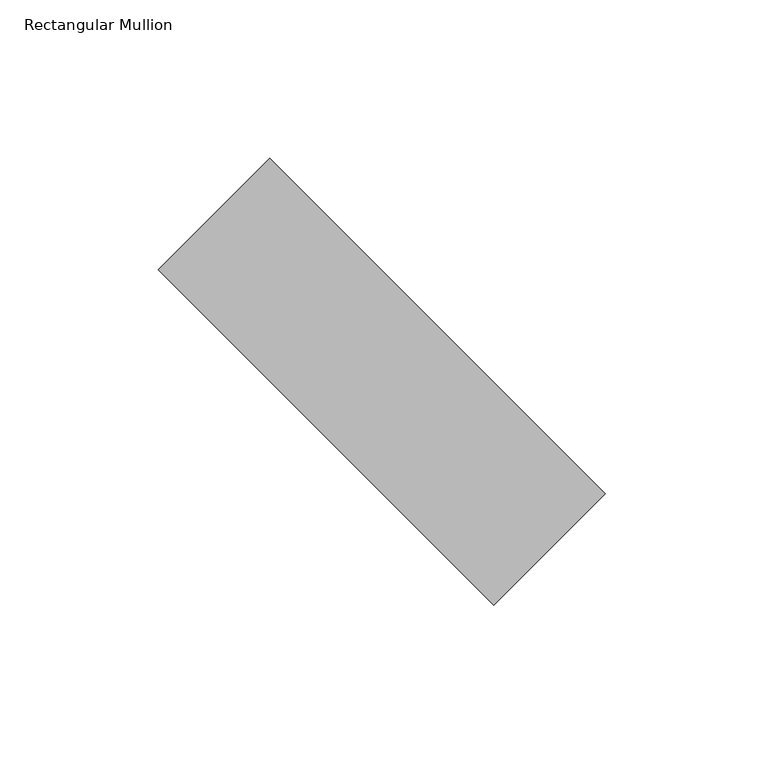
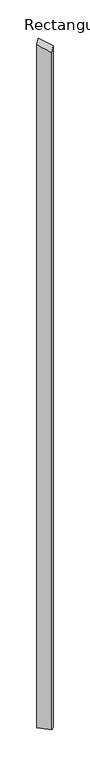
"""IFC4 building model written with IfcOpenShell, lengths in millimetres: member geometry, Rectangular Mullion : tilted mullions."""

from ifc_helpers import new_model, si_unit, origin, place, context, project, spatial, faceted_brep, source, transform, mapped, element, save


def rectangular_mullion_5ef0547a(model_context):
    return source(origin(), model_context, "Body", "Brep", [
        faceted_brep([(-35.3553391, 70.7106781, -7999.4591801), (70.7106781, -35.3553391, -7999.4591801), (35.3553391, -70.7106781, -7999.4591801), (-70.7106781, 35.3553391, -7999.4591801), (-70.7106781, 35.3553391, 9.9989462), (-35.3553391, 70.7106781, 55.052399), (35.3553391, -70.7106781, -55.052399), (70.7106781, -35.3553391, -9.9989462)], [[[0, 1, 2, 3]], [[4, 5, 0, 3]], [[6, 4, 3, 2]], [[7, 6, 2, 1]], [[5, 7, 1, 0]], [[5, 4, 6, 7]]]),
    ])


if __name__ == "__main__":
    model = new_model("IFC4")
    model_context = context("Model", 3, world=origin())
    ifc_project = project(units=[si_unit("LENGTHUNIT", "METRE", prefix="MILLI")], contexts=[model_context])
    site = spatial("IfcSite", under=ifc_project)
    building = spatial("IfcBuilding", under=site)
    placement = place(None, origin())
    rectangular_mullion_shape = rectangular_mullion_5ef0547a(model_context)
    element("IfcMember", 1, ObjectType="Rectangular Mullion : tilted mullions", at=placement, inside=building, context=model_context, shape_type="MappedRepresentation", body=[
        mapped(rectangular_mullion_shape, transform((0.0, 0.0, 0.0), x_axis=(1.0, 0.0, 0.0), y_axis=(0.0, 1.0, 0.0), z_axis=(0.0, 0.0, 1.0))),
    ])
    save(model, "model.ifc")

# Revit data of these elements
# Type "Rectangular Mullion : tilted mullions"
#   built-in parameter 1007304 = 0.492126 (stored number, unit not read)
#   built-in parameter 1007301 = 0.082021 (stored number, unit not read)
#   built-in parameter 1007300 = 0.082021 (stored number, unit not read)
# Element 1 (IfcMember, "Rectangular Mullion : tilted mullions")
#   Materials on its faces: "Aluminum"
# Materials
#   "Aluminum": class "Metal", colour RGB 244 244 244, transparency 0, Description = "Aluminum 6061", Cost = 0
